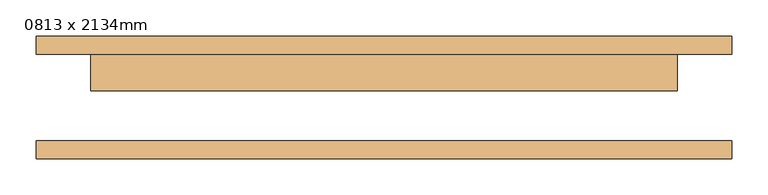
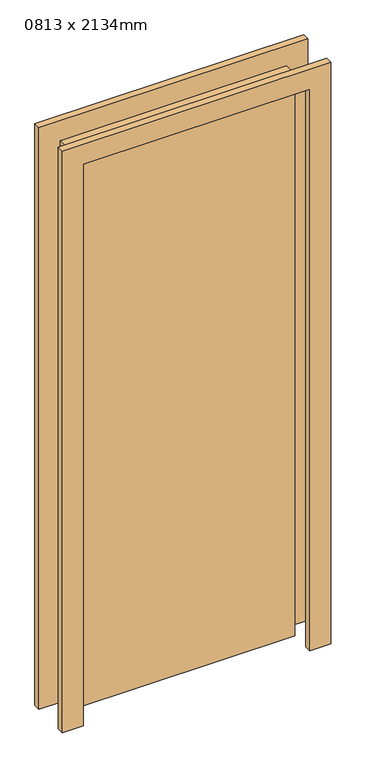
"""IFC4 building model written with IfcOpenShell, lengths in millimetres: door geometry, M_Folha única : 0813 x 2134mm."""

from ifc_helpers import new_model, si_unit, frame, origin, origin_with_axes, place, context, project, spatial, polyline, outline, extrude, source, transform, mapped, element, save


def door_0813_x_2134mm_314d41b2(model_context):
    return source(origin(), model_context, "Body", "SweptSolid", [
        extrude(outline(polyline([(2210.0, -482.5), (0.0, -482.5), (0.0, -406.5), (2134.0, -406.5), (2134.0, 406.5), (0.0, 406.5), (0.0, 482.5), (2210.0, 482.5), (2210.0, -482.5)])), frame((0.0, 60.0, 0.0), z_axis=(0.0, 1.0, 0.0), x_axis=(0.0, 0.0, 1.0)), (0.0, 0.0, 1.0), 25.0),
        extrude(outline(polyline([(2210.0, 482.5), (2210.0, -482.5), (0.0, -482.5), (0.0, -406.5), (2134.0, -406.5), (2134.0, 406.5), (0.0, 406.5), (0.0, 482.5), (2210.0, 482.5)])), frame((0.0, -85.0, 0.0), z_axis=(0.0, 1.0, 0.0), x_axis=(0.0, 0.0, 1.0)), (0.0, 0.0, 1.0), 25.0),
        extrude(outline(polyline([(406.5, 9.0), (-406.5, 9.0), (-406.5, 60.0), (406.5, 60.0), (406.5, 9.0)])), origin_with_axes(), (0.0, 0.0, 1.0), 2134.0),
    ])


if __name__ == "__main__":
    model = new_model("IFC4")
    model_context = context("Model", 3, world=origin())
    ifc_project = project(units=[si_unit("LENGTHUNIT", "METRE", prefix="MILLI")], contexts=[model_context])
    site = spatial("IfcSite", under=ifc_project)
    building = spatial("IfcBuilding", under=site)
    placement = place(None, origin())
    door_0813_x_2134mm_shape = door_0813_x_2134mm_314d41b2(model_context)
    element("IfcDoor", 1, ObjectType="M_Folha única : 0813 x 2134mm", at=placement, inside=building, context=model_context, shape_type="MappedRepresentation", body=[
        mapped(door_0813_x_2134mm_shape, transform((0.0, 0.0, 0.0), x_axis=(1.0, 0.0, 0.0), y_axis=(0.0, 1.0, 0.0), z_axis=(0.0, 0.0, 1.0))),
    ])
    save(model, "model.ifc")

# Revit data of these elements
# Type "M_Folha única : 0813 x 2134mm"
#   Type Mark = "24"
#   Construction Type Id = "MDOOR"
#   Analytic Construction = "Metal"
#   Thickness = 0.051 m
#   Thermal Resistance (R) = 0.270117 (m²·K)/W
#   Heat Transfer Coefficient (U) = 3.7021 W/(m²·K)
#   Height = 2.134 m
#   Projeção da apara externa = 0.025 m
#   Projeção da apara interna = 0.025 m
#   Largura da apara = 0.076 m
#   Width = 0.813 m
#   Define Thermal Properties by = 1
#   Define Thermal Properties by = 1
#   Material da porta = Porta - Painel
#   Material da moldura = Porta - Batente
#   Visual Light Transmittance = 0
#   Solar Heat Gain Coefficient = 0
#   Function = (empty or 0)
#   Wall Closure = (empty or 0)
# Element 1 (IfcDoor, "M_Folha única : 0813 x 2134mm")
#   Materials on its faces: "Porta - Batente", "Porta - Painel"
# Materials
#   "Porta - Painel": class "Madeira", colour RGB 210 159 95, transparency 0, Cost = 0
#   "Porta - Batente": class "Diversos", colour RGB 118 70 51, transparency 0, Cost = 0
